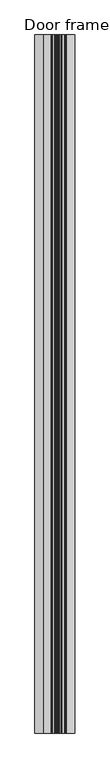
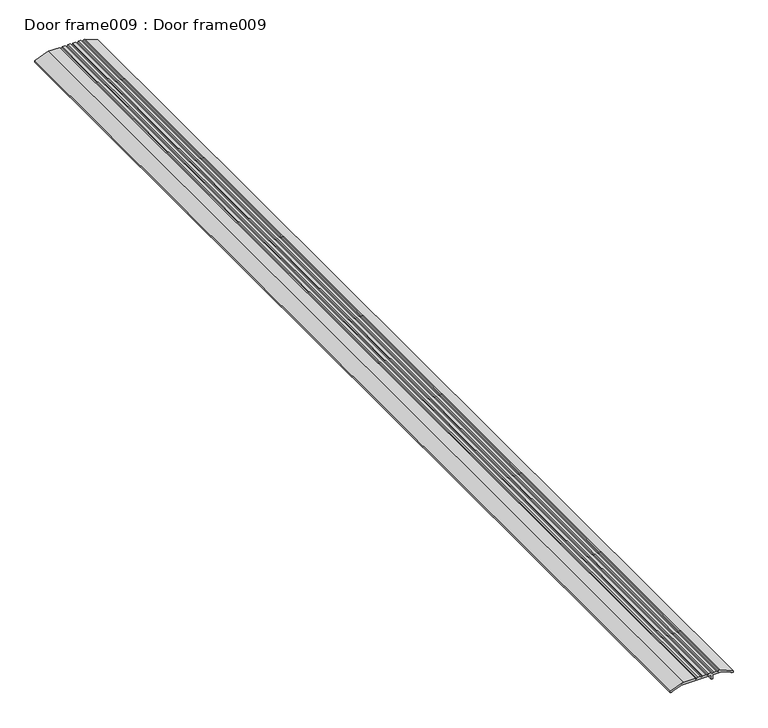
"""IFC4 building model written with IfcOpenShell, lengths in millimetres: proxy geometry, Door frame009 : Door frame009."""

from ifc_helpers import new_model, si_unit, frame, origin, place, context, project, spatial, polyline, outline, extrude, source, transform, mapped, element, save


def door_frame009_door_frame009_747449c1(model_context):
    return source(origin(), model_context, "Body", "SweptSolid", [
        extrude(outline(polyline([(36582.0975353, 15569.2471527), (36582.0975353, 15564.3576527), (36580.0353123, 15563.1670277), (36580.0353123, 15560.7857777), (36582.0975353, 15559.5951527), (36582.0975353, 15554.7056527), (36580.0353123, 15553.5150277), (36580.0353123, 15551.1337777), (36582.0975353, 15549.9431527), (36582.0975353, 15528.6904507), (36572.5243303, 15504.8264027), (36569.3983841, 15504.8264027), (36569.3983841, 15508.0014027), (36570.3770561, 15508.0014027), (36577.3350353, 15525.3462262), (36577.3350353, 15579.7549595), (36569.5937593, 15579.7549595), (36569.5937593, 15582.2978458), (36577.3350353, 15582.2978458), (36577.3350353, 15598.6065792), (36570.3770561, 15615.9514027), (36569.3983841, 15615.9514027), (36569.3983841, 15619.1264027), (36572.5243303, 15619.1264027), (36582.0975353, 15595.2623546), (36582.0975353, 15593.3136527), (36580.0353123, 15592.1230277), (36580.0353123, 15589.7417777), (36582.0975353, 15588.5511527), (36582.0975353, 15583.6616527), (36580.0353123, 15582.4710277), (36580.0353123, 15580.0897777), (36582.0975353, 15578.8991527), (36582.0975353, 15574.0096527), (36580.0353123, 15572.8190277), (36580.0353123, 15570.4377777), (36582.0975353, 15569.2471527)])), frame((0.0, -1052.8906567, 0.0), z_axis=(0.0, 1.0, 0.0), x_axis=(0.0, 0.0, 1.0)), (0.0, 0.0, 1.0), 1999.85),
    ])


if __name__ == "__main__":
    model = new_model("IFC4")
    model_context = context("Model", 3, world=origin())
    ifc_project = project(units=[si_unit("LENGTHUNIT", "METRE", prefix="MILLI")], contexts=[model_context])
    site = spatial("IfcSite", under=ifc_project)
    building = spatial("IfcBuilding", under=site)
    placement = place(None, origin())
    door_frame009_door_frame009_shape = door_frame009_door_frame009_747449c1(model_context)
    element("IfcBuildingElementProxy", 1, Name="Door frame009 : Door frame009", ObjectType="Door frame009 : Door frame009", at=placement, inside=building, context=model_context, shape_type="MappedRepresentation", body=[
        mapped(door_frame009_door_frame009_shape, transform((0.0, 0.0, 0.0), x_axis=(1.0, 0.0, 0.0), y_axis=(0.0, 1.0, 0.0), z_axis=(0.0, 0.0, 1.0))),
    ])
    save(model, "model.ifc")

# Revit data of these elements
# Type "Door frame009 : Door frame009"
#   NameOverride = "Door frame009"
# Element 1 (IfcBuildingElementProxy, "Door frame009 : Door frame009")
#   Materials on its faces: "ALUM. THRESHOLD"
# Materials
#   "ALUM. THRESHOLD": class "Metal", colour RGB 247 247 247, transparency 0, Description = "Aluminum 6061", Cost = 0
